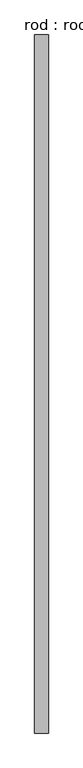
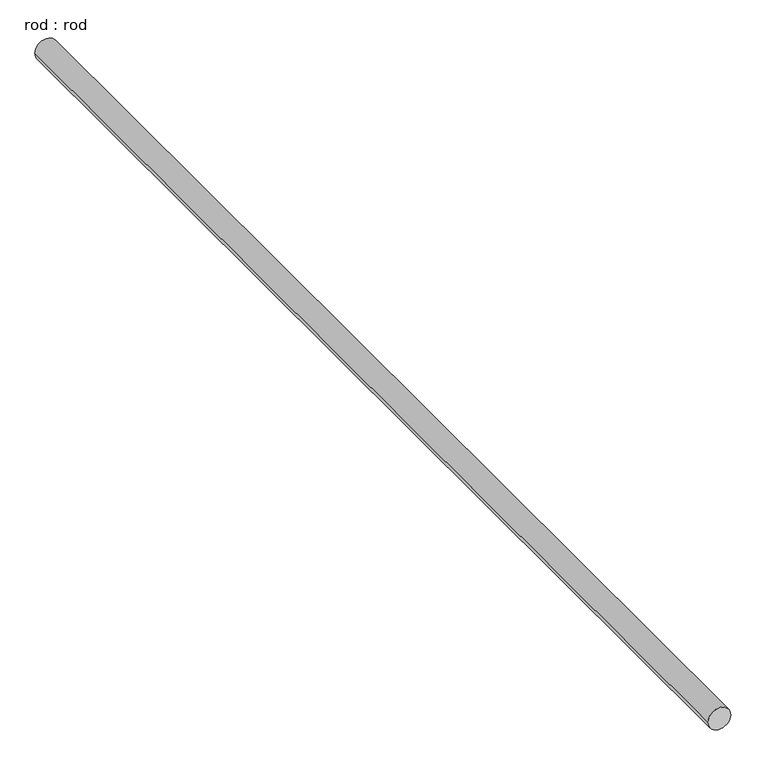
"""IFC4 building model written with IfcOpenShell, lengths in millimetres: proxy geometry, rod : rod."""

import ifcopenshell
import ifcopenshell.guid

model = None  # the IFC model being written
_history = None  # IfcOwnerHistory: only IFC2X3 demands one
_inside = {}  # id of a spatial element -> (the spatial element, [elements in it])
_under = {}  # id of a project, library or spatial element -> (it, [spatial elements below it])
_declared = {}  # id of a project -> (the project, [libraries it declares])
_typed = {}  # id of a type object -> (the type object, [elements of that type])
_made_of = {}  # id of a material, layer set ... -> (it, [elements and type objects made of it])


def new_model(schema):
    """Start an empty IFC model of exactly this schema.

    Asked for "IFC4X3", IfcOpenShell would pick the latest addendum, in which some entities
    have other attributes; the version numbers below select the first issue.
    IFC2X3 requires an IfcOwnerHistory on every rooted entity: one is made here for all.
    """
    global model, _history
    if schema == "IFC4X3":
        model = ifcopenshell.file(schema_version=(4, 3, 0, 0))
    else:
        model = ifcopenshell.file(schema=schema)
    _inside.clear()
    _under.clear()
    _declared.clear()
    _typed.clear()
    _made_of.clear()
    _history = None
    if model.schema == "IFC2X3":
        org = make("IfcOrganization", Name="unknown")
        user = make(
            "IfcPersonAndOrganization",
            ThePerson=make("IfcPerson", FamilyName="unknown"),
            TheOrganization=org,
        )
        app = make(
            "IfcApplication",
            ApplicationDeveloper=org,
            Version="unknown",
            ApplicationFullName="unknown",
            ApplicationIdentifier="unknown",
        )
        _history = make(
            "IfcOwnerHistory",
            OwningUser=user,
            OwningApplication=app,
            ChangeAction="ADDED",
            CreationDate=0,
        )
    return model


def make(cls, **values):
    """One entity of the class cls with the attributes given. An attribute that is None is left unset."""
    return model.create_entity(
        cls, **{name: value for name, value in values.items() if value is not None}
    )


def rooted(cls, **values):
    """An entity with a GlobalId (a new one), such as an element, a storey or a relation."""
    return make(cls, GlobalId=ifcopenshell.guid.new(), OwnerHistory=_history, **values)


def si_unit(unit_type, name, prefix=None):
    """IfcSIUnit, for example si_unit("LENGTHUNIT", "METRE", prefix="MILLI")."""
    return make("IfcSIUnit", UnitType=unit_type, Prefix=prefix, Name=name)


def assignment(units):
    """IfcUnitAssignment: the units of a project."""
    return None if units is None else make("IfcUnitAssignment", Units=units)


def point(xyz):
    """IfcCartesianPoint."""
    return None if xyz is None else make("IfcCartesianPoint", Coordinates=xyz)


def direction(xyz):
    """IfcDirection."""
    return None if xyz is None else make("IfcDirection", DirectionRatios=xyz)


def frame(location, z_axis=None, x_axis=None):
    """IfcAxis2Placement3D, a coordinate frame: its origin and axes. An axis left out is left unset."""
    return make(
        "IfcAxis2Placement3D",
        Location=point(location),
        Axis=direction(z_axis),
        RefDirection=direction(x_axis),
    )


def frame_2d(location, x_axis=None):
    """IfcAxis2Placement2D, a coordinate frame in the plane: its origin and x axis."""
    return make(
        "IfcAxis2Placement2D", Location=point(location), RefDirection=direction(x_axis)
    )


def origin():
    """The frame at (0, 0, 0) with its axes left unset."""
    return frame((0.0, 0.0, 0.0))


def place(relative_to, where):
    """IfcLocalPlacement: puts the frame where relative to a parent placement (None: the world)."""
    return make(
        "IfcLocalPlacement", PlacementRelTo=relative_to, RelativePlacement=where
    )


def context(
    kind, dimensions, precision=None, world=None, true_north=None, identifier=None
):
    """IfcGeometricRepresentationContext, for example the 3D "Model" context."""
    return make(
        "IfcGeometricRepresentationContext",
        ContextIdentifier=identifier,
        ContextType=kind,
        CoordinateSpaceDimension=dimensions,
        Precision=precision,
        WorldCoordinateSystem=world,
        TrueNorth=true_north,
    )


def project(units=None, contexts=None):
    """IfcProject with its units and contexts."""
    return rooted(
        "IfcProject",
        Name="project",
        RepresentationContexts=contexts,
        UnitsInContext=assignment(units),
    )


def spatial(cls, under=None, at=None, **own):
    """A site, building, storey or space (cls), placed at a placement, below another one or the project."""
    s = rooted(cls, ObjectPlacement=at, **own)
    if under is not None:
        _under.setdefault(under.id(), (under, []))[1].append(s)
    return s


def circle_curve(where, radius):
    """IfcCircle in the frame where."""
    return make("IfcCircle", Position=where, Radius=radius)


def trimmed(basis, trim1, trim2, sense, master):
    """IfcTrimmedCurve: the piece of a basis curve between two trims."""
    return make(
        "IfcTrimmedCurve",
        BasisCurve=basis,
        Trim1=trim1,
        Trim2=trim2,
        SenseAgreement=sense,
        MasterRepresentation=master,
    )


def segment(curve, same_sense, transition):
    """IfcCompositeCurveSegment."""
    return make(
        "IfcCompositeCurveSegment",
        Transition=transition,
        SameSense=same_sense,
        ParentCurve=curve,
    )


def composite_curve(segments, self_intersect=None):
    """IfcCompositeCurve: segments joined end to end."""
    return make("IfcCompositeCurve", Segments=segments, SelfIntersect=self_intersect)


def outline(outer, holes=None, kind="AREA"):
    """IfcArbitraryClosedProfileDef: a profile drawn as a closed curve; with holes, ...WithVoids."""
    if holes is None:
        return make("IfcArbitraryClosedProfileDef", ProfileType=kind, OuterCurve=outer)
    return make(
        "IfcArbitraryProfileDefWithVoids",
        ProfileType=kind,
        OuterCurve=outer,
        InnerCurves=holes,
    )


def extrude(swept, where, along, depth):
    """IfcExtrudedAreaSolid: the profile swept, set in the frame where, extruded along a direction by depth."""
    return make(
        "IfcExtrudedAreaSolid",
        SweptArea=swept,
        Position=where,
        ExtrudedDirection=direction(along),
        Depth=depth,
    )


def shape(context_of_items, identifier, shape_type, items):
    """IfcShapeRepresentation: the items that make up one representation, for example the "Body"."""
    return make(
        "IfcShapeRepresentation",
        ContextOfItems=context_of_items,
        RepresentationIdentifier=identifier,
        RepresentationType=shape_type,
        Items=items,
    )


def source(mapping_origin, context_of_items, identifier, shape_type, items):
    """IfcRepresentationMap: a shape defined once, which mapped items show again and again."""
    return make(
        "IfcRepresentationMap",
        MappingOrigin=mapping_origin,
        MappedRepresentation=shape(context_of_items, identifier, shape_type, items),
    )


def transform(
    local_origin,
    x_axis=None,
    y_axis=None,
    z_axis=None,
    scale=None,
    scale2=None,
    scale3=None,
    uniform=True,
):
    """IfcCartesianTransformationOperator3D, or its non-uniform kind. x_axis, y_axis, z_axis: its Axis1, 2, 3."""
    if uniform:
        return make(
            "IfcCartesianTransformationOperator3D",
            Axis1=direction(x_axis),
            Axis2=direction(y_axis),
            LocalOrigin=point(local_origin),
            Scale=scale,
            Axis3=direction(z_axis),
        )
    return make(
        "IfcCartesianTransformationOperator3DnonUniform",
        Axis1=direction(x_axis),
        Axis2=direction(y_axis),
        LocalOrigin=point(local_origin),
        Scale=scale,
        Axis3=direction(z_axis),
        Scale2=scale2,
        Scale3=scale3,
    )


def mapped(mapping_source, mapping_target):
    """IfcMappedItem: shows the shape of a source again, moved by a transform."""
    return make(
        "IfcMappedItem", MappingSource=mapping_source, MappingTarget=mapping_target
    )


def made_of(thing, what):
    """Note that an element or type object is made of a material, layer set ...; save() writes the relation."""
    if what is not None:
        _made_of.setdefault(what.id(), (what, []))[1].append(thing)
    return thing


def element(
    cls,
    number,
    at=None,
    inside=None,
    cuts=None,
    type_object=None,
    material=None,
    context=None,
    identifier="Body",
    shape_type=None,
    held_by="IfcProductDefinitionShape",
    body=None,
    shapes=None,
    **own,
):
    """One element of the class cls, such as IfcWall. Its Tag is "e" and its number.

    at: its placement. inside: the storey or other place that contains it. cuts: it is an
    opening in that element (IfcRelVoidsElement). A single representation is given by context,
    identifier, shape_type and body (its items); several are given by shapes. held_by: the class
    of the entity that holds the representations. save() writes the other relations.
    """
    e = rooted(cls, Tag="e%d" % number, ObjectPlacement=at, **own)
    if body is not None:
        shapes = [shape(context, identifier, shape_type, body)]
    if shapes is not None:
        e.Representation = make(held_by, Representations=shapes)
    if inside is not None:
        _inside.setdefault(inside.id(), (inside, []))[1].append(e)
    if cuts is not None:
        rooted(
            "IfcRelVoidsElement", RelatingBuildingElement=cuts, RelatedOpeningElement=e
        )
    if type_object is not None:
        _typed.setdefault(type_object.id(), (type_object, []))[1].append(e)
    return made_of(e, material)


def aggregate(whole, parts):
    """IfcRelAggregates: a whole, such as a stair, and the parts it consists of."""
    return rooted("IfcRelAggregates", RelatingObject=whole, RelatedObjects=parts)


def save(model, path):
    """Write the relations noted so far, then the file.

    IfcRelAggregates (storeys below a building ...), IfcRelContainedInSpatialStructure (elements
    in a storey), IfcRelDefinesByType, IfcRelAssociatesMaterial and IfcRelDeclares: one each for
    every whole, place, type object, material and project.
    """
    for whole, parts in _under.values():
        aggregate(whole, parts)
    for where, things in _inside.values():
        rooted(
            "IfcRelContainedInSpatialStructure",
            RelatedElements=things,
            RelatingStructure=where,
        )
    for kind, things in _typed.values():
        rooted("IfcRelDefinesByType", RelatedObjects=things, RelatingType=kind)
    for what, things in _made_of.values():
        rooted("IfcRelAssociatesMaterial", RelatedObjects=things, RelatingMaterial=what)
    for by, libraries in _declared.values():
        rooted("IfcRelDeclares", RelatingContext=by, RelatedDefinitions=libraries)
    model.write(path)


def rod_rod_5b1264ed(model_context):
    return source(origin(), model_context, "Body", "SweptSolid", [
        extrude(outline(composite_curve([segment(trimmed(circle_curve(frame_2d((0.0108462, 0.0)), 200.0), [point((0.0108462, 200.0))], [point((0.0108462, -200.0))], False, "CARTESIAN"), True, "CONTINUOUS"), segment(trimmed(circle_curve(frame_2d((0.0108462, 0.0)), 200.0), [point((0.0108462, -200.0))], [point((0.0108462, 200.0))], False, "CARTESIAN"), True, "CONTINUOUS")], self_intersect=False)), frame((0.0, -6157.2713847, 0.0), z_axis=(0.0, 1.0, 0.0), x_axis=(0.0, 0.0, 1.0)), (0.0, 0.0, 1.0), 20500.0),
    ])


if __name__ == "__main__":
    model = new_model("IFC4")
    model_context = context("Model", 3, world=origin())
    ifc_project = project(units=[si_unit("LENGTHUNIT", "METRE", prefix="MILLI")], contexts=[model_context])
    site = spatial("IfcSite", under=ifc_project)
    building = spatial("IfcBuilding", under=site)
    placement = place(None, origin())
    rod_rod_shape = rod_rod_5b1264ed(model_context)
    element("IfcBuildingElementProxy", 1, Name="rod : rod", ObjectType="rod : rod", at=placement, inside=building, context=model_context, shape_type="MappedRepresentation", body=[
        mapped(rod_rod_shape, transform((0.0, 0.0, 0.0), x_axis=(1.0, 0.0, 0.0), y_axis=(0.0, 1.0, 0.0), z_axis=(0.0, 0.0, 1.0))),
    ])
    save(model, "model.ifc")

# Revit data of these elements
# Type "rod : rod"
#   Default Elevation = 0
